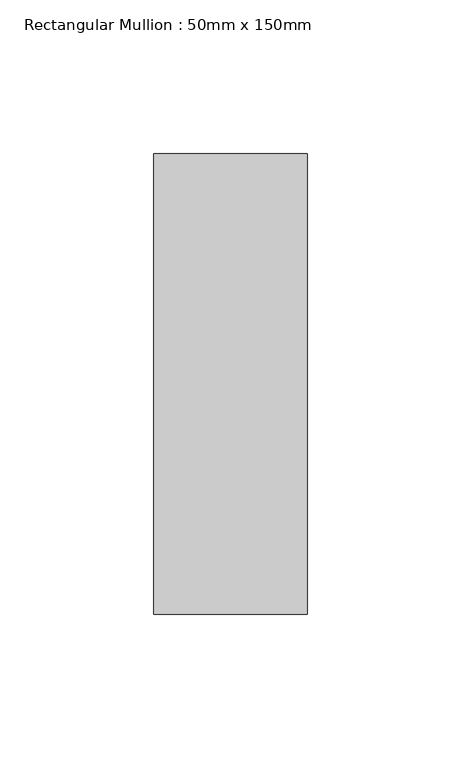
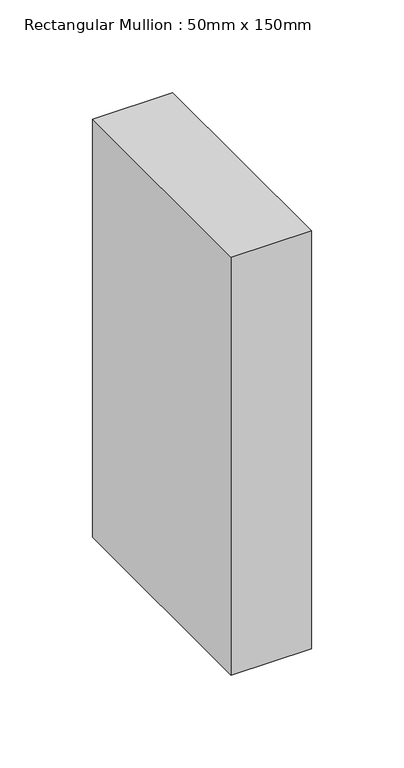
"""IFC4 building model written with IfcOpenShell, lengths in millimetres: member geometry, Rectangular Mullion : 50mm x 150mm."""

from ifc_helpers import new_model, si_unit, frame, origin, place, context, project, spatial, polyline, outline, extrude, source, transform, mapped, element, save


def rectangular_mullion_50mm_x_150mm_2ff57ad4(model_context):
    return source(origin(), model_context, "Body", "SweptSolid", [
        extrude(outline(polyline([(0.0, 75.0), (0.0, -75.0), (-50.0, -75.0), (-50.0, 75.0), (0.0, 75.0)])), frame((0.0, 0.0, -275.7575758), z_axis=(0.0, 0.0, 1.0), x_axis=(1.0, 0.0, 0.0)), (0.0, 0.0, 1.0), 275.7575758),
    ])


if __name__ == "__main__":
    model = new_model("IFC4")
    model_context = context("Model", 3, world=origin())
    ifc_project = project(units=[si_unit("LENGTHUNIT", "METRE", prefix="MILLI")], contexts=[model_context])
    site = spatial("IfcSite", under=ifc_project)
    building = spatial("IfcBuilding", under=site)
    placement = place(None, origin())
    rectangular_mullion_50mm_x_150mm_shape = rectangular_mullion_50mm_x_150mm_2ff57ad4(model_context)
    element("IfcMember", 1, ObjectType="Rectangular Mullion : 50mm x 150mm", at=placement, inside=building, context=model_context, shape_type="MappedRepresentation", body=[
        mapped(rectangular_mullion_50mm_x_150mm_shape, transform((0.0, 0.0, 0.0), x_axis=(1.0, 0.0, 0.0), y_axis=(0.0, 1.0, 0.0), z_axis=(0.0, 0.0, 1.0))),
    ])
    save(model, "model.ifc")

# Revit data of these elements
# Type "Rectangular Mullion : 50mm x 150mm"
#   built-in parameter 1007304 = 0.492126 (stored number, unit not read)
#   built-in parameter 1007301 = 0.082021 (stored number, unit not read)
#   built-in parameter 1007300 = 0.082021 (stored number, unit not read)
# Element 1 (IfcMember, "Rectangular Mullion : 50mm x 150mm")
#   Materials on its faces: "Aluminum"
# Materials
#   "Aluminum": class "Metal", colour RGB 244 244 244, transparency 0, Description = "Aluminum 6061", Cost = 0
